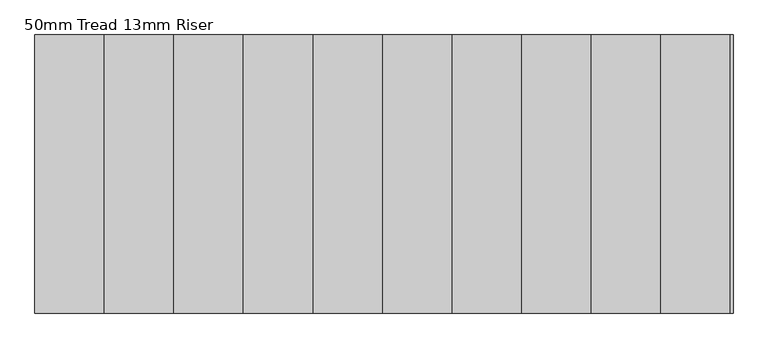
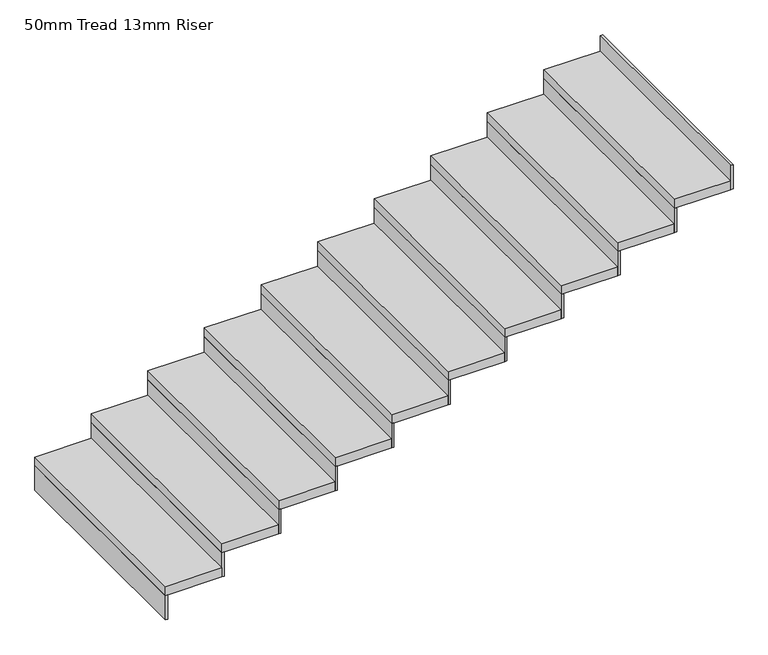
"""IFC4 building model written with IfcOpenShell, lengths in millimetres: stair flight geometry, 50mm Tread 13mm Riser."""

from ifc_helpers import new_model, si_unit, frame, origin, place, context, project, spatial, polyline, outline, extrude, source, transform, mapped, element, save


def stair_flight_50mm_tread_13mm_riser_5a7111b7(model_context):
    return source(origin(), model_context, "Body", "SweptSolid", [
        extrude(outline(polyline([(-7361.9417114, -7269.8807746), (-7374.4417114, -7269.8807746), (-7374.4417114, -6069.8807746), (-7361.9417114, -6069.8807746), (-7361.9417114, -7269.8807746)])), frame((0.0, 0.0, 1450.0), z_axis=(0.0, 0.0, 1.0), x_axis=(1.0, 0.0, 0.0)), (0.0, 0.0, 1.0), 136.3636364),
        extrude(outline(polyline([(-7074.4417114, -6069.8807746), (-7074.4417114, -7269.8807746), (-7374.4417114, -7269.8807746), (-7374.4417114, -6069.8807746), (-7074.4417114, -6069.8807746)])), frame((0.0, 0.0, 1586.3636364), z_axis=(0.0, 0.0, 1.0), x_axis=(1.0, 0.0, 0.0)), (0.0, 0.0, 1.0), 50.0),
        extrude(outline(polyline([(-7061.9417114, -7269.8807746), (-7074.4417114, -7269.8807746), (-7074.4417114, -6069.8807746), (-7061.9417114, -6069.8807746), (-7061.9417114, -7269.8807746)])), frame((0.0, 0.0, 1586.3636364), z_axis=(0.0, 0.0, 1.0), x_axis=(1.0, 0.0, 0.0)), (0.0, 0.0, 1.0), 136.3636364),
        extrude(outline(polyline([(-6774.4417114, -6069.8807746), (-6774.4417114, -7269.8807746), (-7074.4417114, -7269.8807746), (-7074.4417114, -6069.8807746), (-6774.4417114, -6069.8807746)])), frame((0.0, 0.0, 1722.7272727), z_axis=(0.0, 0.0, 1.0), x_axis=(1.0, 0.0, 0.0)), (0.0, 0.0, 1.0), 50.0),
        extrude(outline(polyline([(-6761.9417114, -7269.8807746), (-6774.4417114, -7269.8807746), (-6774.4417114, -6069.8807746), (-6761.9417114, -6069.8807746), (-6761.9417114, -7269.8807746)])), frame((0.0, 0.0, 1722.7272727), z_axis=(0.0, 0.0, 1.0), x_axis=(1.0, 0.0, 0.0)), (0.0, 0.0, 1.0), 136.3636364),
        extrude(outline(polyline([(-6474.4417114, -6069.8807746), (-6474.4417114, -7269.8807746), (-6774.4417114, -7269.8807746), (-6774.4417114, -6069.8807746), (-6474.4417114, -6069.8807746)])), frame((0.0, 0.0, 1859.0909091), z_axis=(0.0, 0.0, 1.0), x_axis=(1.0, 0.0, 0.0)), (0.0, 0.0, 1.0), 50.0),
        extrude(outline(polyline([(-6461.9417114, -7269.8807746), (-6474.4417114, -7269.8807746), (-6474.4417114, -6069.8807746), (-6461.9417114, -6069.8807746), (-6461.9417114, -7269.8807746)])), frame((0.0, 0.0, 1859.0909091), z_axis=(0.0, 0.0, 1.0), x_axis=(1.0, 0.0, 0.0)), (0.0, 0.0, 1.0), 136.3636364),
        extrude(outline(polyline([(-6174.4417114, -6069.8807746), (-6174.4417114, -7269.8807746), (-6474.4417114, -7269.8807746), (-6474.4417114, -6069.8807746), (-6174.4417114, -6069.8807746)])), frame((0.0, 0.0, 1995.4545455), z_axis=(0.0, 0.0, 1.0), x_axis=(1.0, 0.0, 0.0)), (0.0, 0.0, 1.0), 50.0),
        extrude(outline(polyline([(-6161.9417114, -7269.8807746), (-6174.4417114, -7269.8807746), (-6174.4417114, -6069.8807746), (-6161.9417114, -6069.8807746), (-6161.9417114, -7269.8807746)])), frame((0.0, 0.0, 1995.4545455), z_axis=(0.0, 0.0, 1.0), x_axis=(1.0, 0.0, 0.0)), (0.0, 0.0, 1.0), 136.3636364),
        extrude(outline(polyline([(-5874.4417114, -6069.8807746), (-5874.4417114, -7269.8807746), (-6174.4417114, -7269.8807746), (-6174.4417114, -6069.8807746), (-5874.4417114, -6069.8807746)])), frame((0.0, 0.0, 2131.8181818), z_axis=(0.0, 0.0, 1.0), x_axis=(1.0, 0.0, 0.0)), (0.0, 0.0, 1.0), 50.0),
        extrude(outline(polyline([(-5861.9417114, -7269.8807746), (-5874.4417114, -7269.8807746), (-5874.4417114, -6069.8807746), (-5861.9417114, -6069.8807746), (-5861.9417114, -7269.8807746)])), frame((0.0, 0.0, 2131.8181818), z_axis=(0.0, 0.0, 1.0), x_axis=(1.0, 0.0, 0.0)), (0.0, 0.0, 1.0), 136.3636364),
        extrude(outline(polyline([(-5574.4417114, -6069.8807746), (-5574.4417114, -7269.8807746), (-5874.4417114, -7269.8807746), (-5874.4417114, -6069.8807746), (-5574.4417114, -6069.8807746)])), frame((0.0, 0.0, 2268.1818182), z_axis=(0.0, 0.0, 1.0), x_axis=(1.0, 0.0, 0.0)), (0.0, 0.0, 1.0), 50.0),
        extrude(outline(polyline([(-5561.9417114, -7269.8807746), (-5574.4417114, -7269.8807746), (-5574.4417114, -6069.8807746), (-5561.9417114, -6069.8807746), (-5561.9417114, -7269.8807746)])), frame((0.0, 0.0, 2268.1818182), z_axis=(0.0, 0.0, 1.0), x_axis=(1.0, 0.0, 0.0)), (0.0, 0.0, 1.0), 136.3636364),
        extrude(outline(polyline([(-5274.4417114, -6069.8807746), (-5274.4417114, -7269.8807746), (-5574.4417114, -7269.8807746), (-5574.4417114, -6069.8807746), (-5274.4417114, -6069.8807746)])), frame((0.0, 0.0, 2404.5454545), z_axis=(0.0, 0.0, 1.0), x_axis=(1.0, 0.0, 0.0)), (0.0, 0.0, 1.0), 50.0),
        extrude(outline(polyline([(-5261.9417114, -7269.8807746), (-5274.4417114, -7269.8807746), (-5274.4417114, -6069.8807746), (-5261.9417114, -6069.8807746), (-5261.9417114, -7269.8807746)])), frame((0.0, 0.0, 2404.5454545), z_axis=(0.0, 0.0, 1.0), x_axis=(1.0, 0.0, 0.0)), (0.0, 0.0, 1.0), 136.3636364),
        extrude(outline(polyline([(-4974.4417114, -6069.8807746), (-4974.4417114, -7269.8807746), (-5274.4417114, -7269.8807746), (-5274.4417114, -6069.8807746), (-4974.4417114, -6069.8807746)])), frame((0.0, 0.0, 2540.9090909), z_axis=(0.0, 0.0, 1.0), x_axis=(1.0, 0.0, 0.0)), (0.0, 0.0, 1.0), 50.0),
        extrude(outline(polyline([(-4961.9417114, -7269.8807746), (-4974.4417114, -7269.8807746), (-4974.4417114, -6069.8807746), (-4961.9417114, -6069.8807746), (-4961.9417114, -7269.8807746)])), frame((0.0, 0.0, 2540.9090909), z_axis=(0.0, 0.0, 1.0), x_axis=(1.0, 0.0, 0.0)), (0.0, 0.0, 1.0), 136.3636364),
        extrude(outline(polyline([(-4674.4417114, -6069.8807746), (-4674.4417114, -7269.8807746), (-4974.4417114, -7269.8807746), (-4974.4417114, -6069.8807746), (-4674.4417114, -6069.8807746)])), frame((0.0, 0.0, 2677.2727273), z_axis=(0.0, 0.0, 1.0), x_axis=(1.0, 0.0, 0.0)), (0.0, 0.0, 1.0), 50.0),
        extrude(outline(polyline([(-4661.9417114, -7269.8807746), (-4674.4417114, -7269.8807746), (-4674.4417114, -6069.8807746), (-4661.9417114, -6069.8807746), (-4661.9417114, -7269.8807746)])), frame((0.0, 0.0, 2677.2727273), z_axis=(0.0, 0.0, 1.0), x_axis=(1.0, 0.0, 0.0)), (0.0, 0.0, 1.0), 136.3636364),
        extrude(outline(polyline([(-4361.9417114, -7269.8807746), (-4374.4417114, -7269.8807746), (-4374.4417114, -6069.8807746), (-4361.9417114, -6069.8807746), (-4361.9417114, -7269.8807746)])), frame((0.0, 0.0, 2813.6363636), z_axis=(0.0, 0.0, 1.0), x_axis=(1.0, 0.0, 0.0)), (0.0, 0.0, 1.0), 136.3636364),
        extrude(outline(polyline([(-4374.4417114, -6069.8807746), (-4374.4417114, -7269.8807746), (-4674.4417114, -7269.8807746), (-4674.4417114, -6069.8807746), (-4374.4417114, -6069.8807746)])), frame((0.0, 0.0, 2813.6363636), z_axis=(0.0, 0.0, 1.0), x_axis=(1.0, 0.0, 0.0)), (0.0, 0.0, 1.0), 50.0),
    ])


if __name__ == "__main__":
    model = new_model("IFC4")
    model_context = context("Model", 3, world=origin())
    ifc_project = project(units=[si_unit("LENGTHUNIT", "METRE", prefix="MILLI")], contexts=[model_context])
    site = spatial("IfcSite", under=ifc_project)
    building = spatial("IfcBuilding", under=site)
    placement = place(None, origin())
    stair_flight_50mm_tread_13mm_riser_shape = stair_flight_50mm_tread_13mm_riser_5a7111b7(model_context)
    element("IfcStairFlight", 1, ObjectType="50mm Tread 13mm Riser", at=placement, inside=building, context=model_context, shape_type="MappedRepresentation", body=[
        mapped(stair_flight_50mm_tread_13mm_riser_shape, transform((0.0, 0.0, 0.0), x_axis=(1.0, 0.0, 0.0), y_axis=(0.0, 1.0, 0.0), z_axis=(0.0, 0.0, 1.0))),
    ])
    save(model, "model.ifc")

# Revit data of these elements
# Project information
#   Project Issue Date = "Issue Date"
#   Project Status = "Project Status"
#   Client Name = "Owner"
#   Project Address = "Enter address here"
#   Project Name = "Project Name"
#   Project Number = "0001"
